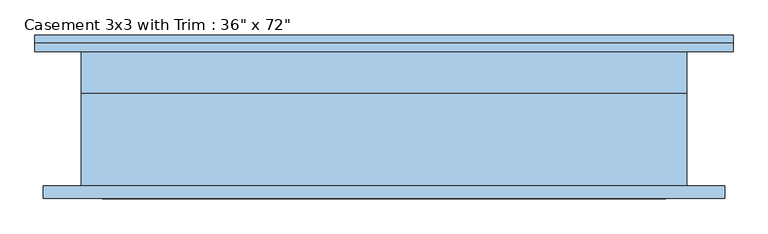
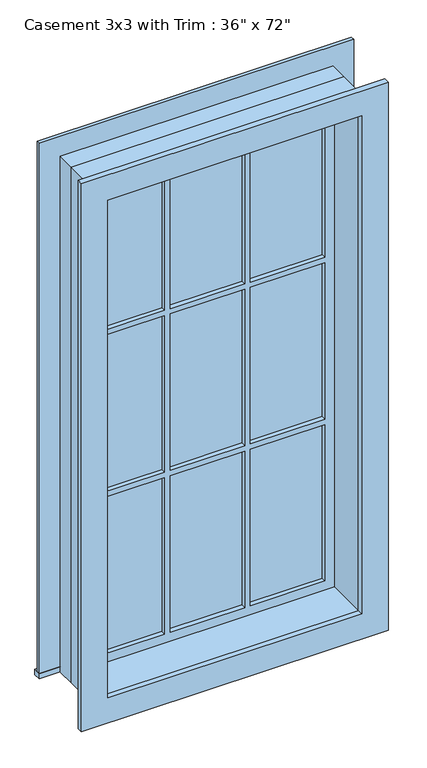
"""IFC4 building model written with IfcOpenShell, lengths in millimetres: window geometry."""

import ifcopenshell
import ifcopenshell.guid

model = None  # the IFC model being written
_history = None  # IfcOwnerHistory: only IFC2X3 demands one
_inside = {}  # id of a spatial element -> (the spatial element, [elements in it])
_under = {}  # id of a project, library or spatial element -> (it, [spatial elements below it])
_declared = {}  # id of a project -> (the project, [libraries it declares])
_typed = {}  # id of a type object -> (the type object, [elements of that type])
_made_of = {}  # id of a material, layer set ... -> (it, [elements and type objects made of it])


def new_model(schema):
    """Start an empty IFC model of exactly this schema.

    Asked for "IFC4X3", IfcOpenShell would pick the latest addendum, in which some entities
    have other attributes; the version numbers below select the first issue.
    IFC2X3 requires an IfcOwnerHistory on every rooted entity: one is made here for all.
    """
    global model, _history
    if schema == "IFC4X3":
        model = ifcopenshell.file(schema_version=(4, 3, 0, 0))
    else:
        model = ifcopenshell.file(schema=schema)
    _inside.clear()
    _under.clear()
    _declared.clear()
    _typed.clear()
    _made_of.clear()
    _history = None
    if model.schema == "IFC2X3":
        org = make("IfcOrganization", Name="unknown")
        user = make(
            "IfcPersonAndOrganization",
            ThePerson=make("IfcPerson", FamilyName="unknown"),
            TheOrganization=org,
        )
        app = make(
            "IfcApplication",
            ApplicationDeveloper=org,
            Version="unknown",
            ApplicationFullName="unknown",
            ApplicationIdentifier="unknown",
        )
        _history = make(
            "IfcOwnerHistory",
            OwningUser=user,
            OwningApplication=app,
            ChangeAction="ADDED",
            CreationDate=0,
        )
    return model


def make(cls, **values):
    """One entity of the class cls with the attributes given. An attribute that is None is left unset."""
    return model.create_entity(
        cls, **{name: value for name, value in values.items() if value is not None}
    )


def rooted(cls, **values):
    """An entity with a GlobalId (a new one), such as an element, a storey or a relation."""
    return make(cls, GlobalId=ifcopenshell.guid.new(), OwnerHistory=_history, **values)


def si_unit(unit_type, name, prefix=None):
    """IfcSIUnit, for example si_unit("LENGTHUNIT", "METRE", prefix="MILLI")."""
    return make("IfcSIUnit", UnitType=unit_type, Prefix=prefix, Name=name)


def assignment(units):
    """IfcUnitAssignment: the units of a project."""
    return None if units is None else make("IfcUnitAssignment", Units=units)


def point(xyz):
    """IfcCartesianPoint."""
    return None if xyz is None else make("IfcCartesianPoint", Coordinates=xyz)


def direction(xyz):
    """IfcDirection."""
    return None if xyz is None else make("IfcDirection", DirectionRatios=xyz)


def frame(location, z_axis=None, x_axis=None):
    """IfcAxis2Placement3D, a coordinate frame: its origin and axes. An axis left out is left unset."""
    return make(
        "IfcAxis2Placement3D",
        Location=point(location),
        Axis=direction(z_axis),
        RefDirection=direction(x_axis),
    )


def origin():
    """The frame at (0, 0, 0) with its axes left unset."""
    return frame((0.0, 0.0, 0.0))


def place(relative_to, where):
    """IfcLocalPlacement: puts the frame where relative to a parent placement (None: the world)."""
    return make(
        "IfcLocalPlacement", PlacementRelTo=relative_to, RelativePlacement=where
    )


def context(
    kind, dimensions, precision=None, world=None, true_north=None, identifier=None
):
    """IfcGeometricRepresentationContext, for example the 3D "Model" context."""
    return make(
        "IfcGeometricRepresentationContext",
        ContextIdentifier=identifier,
        ContextType=kind,
        CoordinateSpaceDimension=dimensions,
        Precision=precision,
        WorldCoordinateSystem=world,
        TrueNorth=true_north,
    )


def project(units=None, contexts=None):
    """IfcProject with its units and contexts."""
    return rooted(
        "IfcProject",
        Name="project",
        RepresentationContexts=contexts,
        UnitsInContext=assignment(units),
    )


def spatial(cls, under=None, at=None, **own):
    """A site, building, storey or space (cls), placed at a placement, below another one or the project."""
    s = rooted(cls, ObjectPlacement=at, **own)
    if under is not None:
        _under.setdefault(under.id(), (under, []))[1].append(s)
    return s


def polyline(points):
    """IfcPolyline through the points."""
    return make("IfcPolyline", Points=[point(p) for p in points])


def outline(outer, holes=None, kind="AREA"):
    """IfcArbitraryClosedProfileDef: a profile drawn as a closed curve; with holes, ...WithVoids."""
    if holes is None:
        return make("IfcArbitraryClosedProfileDef", ProfileType=kind, OuterCurve=outer)
    return make(
        "IfcArbitraryProfileDefWithVoids",
        ProfileType=kind,
        OuterCurve=outer,
        InnerCurves=holes,
    )


def extrude(swept, where, along, depth):
    """IfcExtrudedAreaSolid: the profile swept, set in the frame where, extruded along a direction by depth."""
    return make(
        "IfcExtrudedAreaSolid",
        SweptArea=swept,
        Position=where,
        ExtrudedDirection=direction(along),
        Depth=depth,
    )


def shape(context_of_items, identifier, shape_type, items):
    """IfcShapeRepresentation: the items that make up one representation, for example the "Body"."""
    return make(
        "IfcShapeRepresentation",
        ContextOfItems=context_of_items,
        RepresentationIdentifier=identifier,
        RepresentationType=shape_type,
        Items=items,
    )


def source(mapping_origin, context_of_items, identifier, shape_type, items):
    """IfcRepresentationMap: a shape defined once, which mapped items show again and again."""
    return make(
        "IfcRepresentationMap",
        MappingOrigin=mapping_origin,
        MappedRepresentation=shape(context_of_items, identifier, shape_type, items),
    )


def transform(
    local_origin,
    x_axis=None,
    y_axis=None,
    z_axis=None,
    scale=None,
    scale2=None,
    scale3=None,
    uniform=True,
):
    """IfcCartesianTransformationOperator3D, or its non-uniform kind. x_axis, y_axis, z_axis: its Axis1, 2, 3."""
    if uniform:
        return make(
            "IfcCartesianTransformationOperator3D",
            Axis1=direction(x_axis),
            Axis2=direction(y_axis),
            LocalOrigin=point(local_origin),
            Scale=scale,
            Axis3=direction(z_axis),
        )
    return make(
        "IfcCartesianTransformationOperator3DnonUniform",
        Axis1=direction(x_axis),
        Axis2=direction(y_axis),
        LocalOrigin=point(local_origin),
        Scale=scale,
        Axis3=direction(z_axis),
        Scale2=scale2,
        Scale3=scale3,
    )


def mapped(mapping_source, mapping_target):
    """IfcMappedItem: shows the shape of a source again, moved by a transform."""
    return make(
        "IfcMappedItem", MappingSource=mapping_source, MappingTarget=mapping_target
    )


def made_of(thing, what):
    """Note that an element or type object is made of a material, layer set ...; save() writes the relation."""
    if what is not None:
        _made_of.setdefault(what.id(), (what, []))[1].append(thing)
    return thing


def element(
    cls,
    number,
    at=None,
    inside=None,
    cuts=None,
    type_object=None,
    material=None,
    context=None,
    identifier="Body",
    shape_type=None,
    held_by="IfcProductDefinitionShape",
    body=None,
    shapes=None,
    **own,
):
    """One element of the class cls, such as IfcWall. Its Tag is "e" and its number.

    at: its placement. inside: the storey or other place that contains it. cuts: it is an
    opening in that element (IfcRelVoidsElement). A single representation is given by context,
    identifier, shape_type and body (its items); several are given by shapes. held_by: the class
    of the entity that holds the representations. save() writes the other relations.
    """
    e = rooted(cls, Tag="e%d" % number, ObjectPlacement=at, **own)
    if body is not None:
        shapes = [shape(context, identifier, shape_type, body)]
    if shapes is not None:
        e.Representation = make(held_by, Representations=shapes)
    if inside is not None:
        _inside.setdefault(inside.id(), (inside, []))[1].append(e)
    if cuts is not None:
        rooted(
            "IfcRelVoidsElement", RelatingBuildingElement=cuts, RelatedOpeningElement=e
        )
    if type_object is not None:
        _typed.setdefault(type_object.id(), (type_object, []))[1].append(e)
    return made_of(e, material)


def aggregate(whole, parts):
    """IfcRelAggregates: a whole, such as a stair, and the parts it consists of."""
    return rooted("IfcRelAggregates", RelatingObject=whole, RelatedObjects=parts)


def save(model, path):
    """Write the relations noted so far, then the file.

    IfcRelAggregates (storeys below a building ...), IfcRelContainedInSpatialStructure (elements
    in a storey), IfcRelDefinesByType, IfcRelAssociatesMaterial and IfcRelDeclares: one each for
    every whole, place, type object, material and project.
    """
    for whole, parts in _under.values():
        aggregate(whole, parts)
    for where, things in _inside.values():
        rooted(
            "IfcRelContainedInSpatialStructure",
            RelatedElements=things,
            RelatingStructure=where,
        )
    for kind, things in _typed.values():
        rooted("IfcRelDefinesByType", RelatedObjects=things, RelatingType=kind)
    for what, things in _made_of.values():
        rooted("IfcRelAssociatesMaterial", RelatedObjects=things, RelatingMaterial=what)
    for by, libraries in _declared.values():
        rooted("IfcRelDeclares", RelatingContext=by, RelatedDefinitions=libraries)
    model.write(path)


def window_8b323df3(model_context):
    return source(origin(), model_context, "Body", "SweptSolid", [
        extrude(outline(polyline([(-527.05, 127.0), (527.05, 127.0), (527.05, 101.6), (-527.05, 101.6), (-527.05, 127.0)])), frame((0.0, 0.0, 304.8), z_axis=(0.0, 0.0, 1.0), x_axis=(1.0, 0.0, 0.0)), (0.0, 0.0, 1.0), 19.05),
        extrude(outline(polyline([(2114.55, -438.15), (2114.55, 438.15), (323.85, 438.15), (323.85, 527.05), (2203.45, 527.05), (2203.45, -527.05), (323.85, -527.05), (323.85, -438.15), (2114.55, -438.15)])), frame((0.0, 101.6, 0.0), z_axis=(0.0, 1.0, 0.0), x_axis=(0.0, 0.0, 1.0)), (0.0, 0.0, 1.0), 12.7),
        extrude(outline(polyline([(143.9333333, 66.675), (393.7, 66.675), (393.7, 53.975), (143.9333333, 53.975), (143.9333333, 66.675)])), frame((0.0, 0.0, 1515.5333333), z_axis=(0.0, 0.0, 1.0), x_axis=(1.0, 0.0, 0.0)), (0.0, 0.0, 1.0), 554.5666667),
        extrude(outline(polyline([(-124.8833333, 66.675), (124.8833333, 66.675), (124.8833333, 53.975), (-124.8833333, 53.975), (-124.8833333, 66.675)])), frame((0.0, 0.0, 1515.5333333), z_axis=(0.0, 0.0, 1.0), x_axis=(1.0, 0.0, 0.0)), (0.0, 0.0, 1.0), 554.5666667),
        extrude(outline(polyline([(-393.7, 66.675), (-143.9333333, 66.675), (-143.9333333, 53.975), (-393.7, 53.975), (-393.7, 66.675)])), frame((0.0, 0.0, 1515.5333333), z_axis=(0.0, 0.0, 1.0), x_axis=(1.0, 0.0, 0.0)), (0.0, 0.0, 1.0), 554.5666667),
        extrude(outline(polyline([(-393.7, 66.675), (-143.9333333, 66.675), (-143.9333333, 53.975), (-393.7, 53.975), (-393.7, 66.675)])), frame((0.0, 0.0, 941.9166667), z_axis=(0.0, 0.0, 1.0), x_axis=(1.0, 0.0, 0.0)), (0.0, 0.0, 1.0), 554.5666667),
        extrude(outline(polyline([(-124.8833333, 66.675), (124.8833333, 66.675), (124.8833333, 53.975), (-124.8833333, 53.975), (-124.8833333, 66.675)])), frame((0.0, 0.0, 941.9166667), z_axis=(0.0, 0.0, 1.0), x_axis=(1.0, 0.0, 0.0)), (0.0, 0.0, 1.0), 554.5666667),
        extrude(outline(polyline([(143.9333333, 66.675), (393.7, 66.675), (393.7, 53.975), (143.9333333, 53.975), (143.9333333, 66.675)])), frame((0.0, 0.0, 941.9166667), z_axis=(0.0, 0.0, 1.0), x_axis=(1.0, 0.0, 0.0)), (0.0, 0.0, 1.0), 554.5666667),
        extrude(outline(polyline([(143.9333333, 66.675), (393.7, 66.675), (393.7, 53.975), (143.9333333, 53.975), (143.9333333, 66.675)])), frame((0.0, 0.0, 368.3), z_axis=(0.0, 0.0, 1.0), x_axis=(1.0, 0.0, 0.0)), (0.0, 0.0, 1.0), 554.5666667),
        extrude(outline(polyline([(-124.8833333, 66.675), (124.8833333, 66.675), (124.8833333, 53.975), (-124.8833333, 53.975), (-124.8833333, 66.675)])), frame((0.0, 0.0, 368.3), z_axis=(0.0, 0.0, 1.0), x_axis=(1.0, 0.0, 0.0)), (0.0, 0.0, 1.0), 554.5666667),
        extrude(outline(polyline([(-393.7, 66.675), (-143.9333333, 66.675), (-143.9333333, 53.975), (-393.7, 53.975), (-393.7, 66.675)])), frame((0.0, 0.0, 368.3), z_axis=(0.0, 0.0, 1.0), x_axis=(1.0, 0.0, 0.0)), (0.0, 0.0, 1.0), 554.5666667),
        extrude(outline(polyline([(2190.75, 514.35), (2190.75, -514.35), (247.65, -514.35), (247.65, 514.35), (2190.75, 514.35)]), holes=[polyline([(2101.85, 425.45), (336.55, 425.45), (336.55, -425.45), (2101.85, -425.45), (2101.85, 425.45)])]), frame((0.0, -120.65, 0.0), z_axis=(0.0, 1.0, 0.0), x_axis=(0.0, 0.0, 1.0)), (0.0, 0.0, 1.0), 19.05),
        extrude(outline(polyline([(2114.55, -438.15), (323.85, -438.15), (323.85, 438.15), (2114.55, 438.15), (2114.55, -438.15)]), holes=[polyline([(2070.1, -143.9333333), (1515.5333333, -143.9333333), (1515.5333333, -393.7), (2070.1, -393.7), (2070.1, -143.9333333)]), polyline([(1496.4833333, -143.9333333), (941.9166667, -143.9333333), (941.9166667, -393.7), (1496.4833333, -393.7), (1496.4833333, -143.9333333)]), polyline([(922.8666667, -143.9333333), (368.3, -143.9333333), (368.3, -393.7), (922.8666667, -393.7), (922.8666667, -143.9333333)]), polyline([(2070.1, 124.8833333), (1515.5333333, 124.8833333), (1515.5333333, -124.8833333), (2070.1, -124.8833333), (2070.1, 124.8833333)]), polyline([(1496.4833333, 124.8833333), (941.9166667, 124.8833333), (941.9166667, -124.8833333), (1496.4833333, -124.8833333), (1496.4833333, 124.8833333)]), polyline([(922.8666667, 124.8833333), (368.3, 124.8833333), (368.3, -124.8833333), (922.8666667, -124.8833333), (922.8666667, 124.8833333)]), polyline([(2070.1, 393.7), (1515.5333333, 393.7), (1515.5333333, 143.9333333), (2070.1, 143.9333333), (2070.1, 393.7)]), polyline([(1496.4833333, 393.7), (941.9166667, 393.7), (941.9166667, 143.9333333), (1496.4833333, 143.9333333), (1496.4833333, 393.7)]), polyline([(922.8666667, 393.7), (368.3, 393.7), (368.3, 143.9333333), (922.8666667, 143.9333333), (922.8666667, 393.7)])]), frame((0.0, 38.1, 0.0), z_axis=(0.0, 1.0, 0.0), x_axis=(0.0, 0.0, 1.0)), (0.0, 0.0, 1.0), 44.45),
        extrude(outline(polyline([(2133.6, -457.2), (304.8, -457.2), (304.8, 457.2), (2133.6, 457.2), (2133.6, -457.2)]), holes=[polyline([(2101.85, -425.45), (2101.85, 425.45), (336.55, 425.45), (336.55, -425.45), (2101.85, -425.45)])]), frame((0.0, -101.6, 0.0), z_axis=(0.0, 1.0, 0.0), x_axis=(0.0, 0.0, 1.0)), (0.0, 0.0, 1.0), 139.7),
        extrude(outline(polyline([(2133.6, 457.2), (2133.6, -457.2), (304.8, -457.2), (304.8, 457.2), (2133.6, 457.2)]), holes=[polyline([(2114.55, 438.15), (323.85, 438.15), (323.85, -438.15), (2114.55, -438.15), (2114.55, 438.15)])]), frame((0.0, 38.1, 0.0), z_axis=(0.0, 1.0, 0.0), x_axis=(0.0, 0.0, 1.0)), (0.0, 0.0, 1.0), 63.5),
    ])


if __name__ == "__main__":
    model = new_model("IFC4")
    model_context = context("Model", 3, world=origin())
    ifc_project = project(units=[si_unit("LENGTHUNIT", "METRE", prefix="MILLI")], contexts=[model_context])
    site = spatial("IfcSite", under=ifc_project)
    building = spatial("IfcBuilding", under=site)
    placement = place(None, origin())
    window_shape = window_8b323df3(model_context)
    element("IfcWindow", 1, ObjectType="Casement 3x3 with Trim : 36\" x 72\"", at=placement, inside=building, context=model_context, shape_type="MappedRepresentation", body=[
        mapped(window_shape, transform((0.0, 0.0, 0.0), x_axis=(1.0, 0.0, 0.0), y_axis=(0.0, 1.0, 0.0), z_axis=(0.0, 0.0, 1.0))),
    ])
    save(model, "model.ifc")

# Revit data of these elements
# Type "Casement 3x3 with Trim : 36\" x 72\""
#   Type Mark = "28"
#   Construction Type Id = "GSP4R"
#   Assembly Code = "B2020100"
#   Analytic Construction = "1/8 in Pilkington single glazing"
#   Visual Light Transmittance = 0.9
#   Solar Heat Gain Coefficient = 0.78
#   Heat Transfer Coefficient (U) = 3.6886 W/(m²·K)
#   Height = 6' - 0"
#   Default Sill Height = 1' - 0"
#   Trim Projection - Ext. = 0' - 0 1/2"
#   Trim Projection - Int. = 0' - 0 3/4"
#   Trim Width - Exterior = 0' - 3 1/2"
#   Trim Width - Interior = 0' - 3 1/2"
#   Width = 3' - 0"
#   Window Inset = 0' - 0 3/4"
#   Glass Pane Material = Glass
#   Sash Material = Sash
#   Trim Exterior Material = Trim
#   Trim Interior Material = Trim
#   Wall Closure = (empty or 0)
# Element 1 (IfcWindow, "Casement 3x3 with Trim : 36\" x 72\"")
#   Materials on its faces: "Sash", "Glass", "Trim"
# Materials
#   "Glass": class "Glass", colour RGB 0 128 192, transparency 0.75, Description = "Soda Lime Glass", Cost = 0
#   "Sash": class "Wood", colour RGB 224 178 126, transparency 0, Cost = 0
#   "Trim": class "Wood", colour RGB 224 178 126, transparency 0
